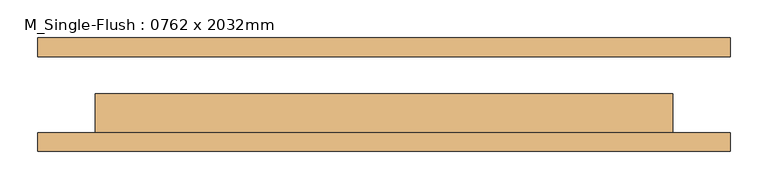
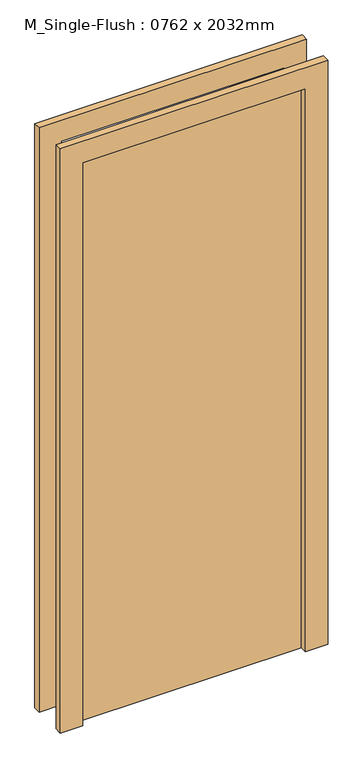
"""IFC4 building model written with IfcOpenShell, lengths in millimetres: door geometry, M_Single-Flush : 0762 x 2032mm."""

from ifc_helpers import new_model, si_unit, frame, origin, origin_with_axes, place, context, project, spatial, polyline, outline, extrude, source, transform, mapped, element, save


def m_single_flush_0762_x_2032mm_fe61752d(model_context):
    return source(origin(), model_context, "Body", "SweptSolid", [
        extrude(outline(polyline([(2108.0, -457.0), (0.0, -457.0), (0.0, -381.0), (2032.0, -381.0), (2032.0, 381.0), (0.0, 381.0), (0.0, 457.0), (2108.0, 457.0), (2108.0, -457.0)])), frame((0.0, -75.0, 0.0), z_axis=(0.0, 1.0, 0.0), x_axis=(0.0, 0.0, 1.0)), (0.0, 0.0, 1.0), 25.0),
        extrude(outline(polyline([(2108.0, 457.0), (2108.0, -457.0), (0.0, -457.0), (0.0, -381.0), (2032.0, -381.0), (2032.0, 381.0), (0.0, 381.0), (0.0, 457.0), (2108.0, 457.0)])), frame((0.0, 50.0, 0.0), z_axis=(0.0, 1.0, 0.0), x_axis=(0.0, 0.0, 1.0)), (0.0, 0.0, 1.0), 25.0),
        extrude(outline(polyline([(381.0, 1.0), (381.0, -50.0), (-381.0, -50.0), (-381.0, 1.0), (381.0, 1.0)])), origin_with_axes(), (0.0, 0.0, 1.0), 2032.0),
    ])


if __name__ == "__main__":
    model = new_model("IFC4")
    model_context = context("Model", 3, world=origin())
    ifc_project = project(units=[si_unit("LENGTHUNIT", "METRE", prefix="MILLI")], contexts=[model_context])
    site = spatial("IfcSite", under=ifc_project)
    building = spatial("IfcBuilding", under=site)
    placement = place(None, origin())
    m_single_flush_0762_x_2032mm_shape = m_single_flush_0762_x_2032mm_fe61752d(model_context)
    element("IfcDoor", 1, ObjectType="M_Single-Flush : 0762 x 2032mm", at=placement, inside=building, context=model_context, shape_type="MappedRepresentation", body=[
        mapped(m_single_flush_0762_x_2032mm_shape, transform((0.0, 0.0, 0.0), x_axis=(1.0, 0.0, 0.0), y_axis=(0.0, 1.0, 0.0), z_axis=(0.0, 0.0, 1.0))),
    ])
    save(model, "model.ifc")

# Revit data of these elements
# Type "M_Single-Flush : 0762 x 2032mm"
#   Type Mark = "19"
#   Thickness = 0.051 m
#   Height = 2.032 m
#   Trim Projection Ext = 0.025 m
#   Trim Projection Int = 0.025 m
#   Trim Width = 0.076 m
#   Width = 0.762 m
#   Door Material = Door - Panel
#   Frame Material = Door - Frame
#   Function = (empty or 0)
#   Wall Closure = (empty or 0)
# Element 1 (IfcDoor, "M_Single-Flush : 0762 x 2032mm")
#   Materials on its faces: "Door - Frame", "Door - Panel"
# Materials
#   "Door - Panel": class "Wood", colour RGB 114 82 51, transparency 0
#   "Door - Frame": class "Miscellaneous", colour RGB 153 76 43, transparency 0
